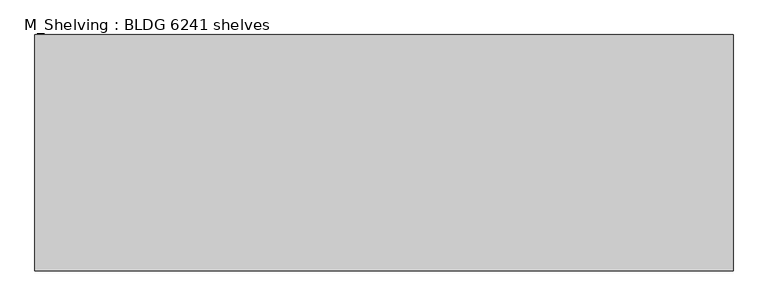
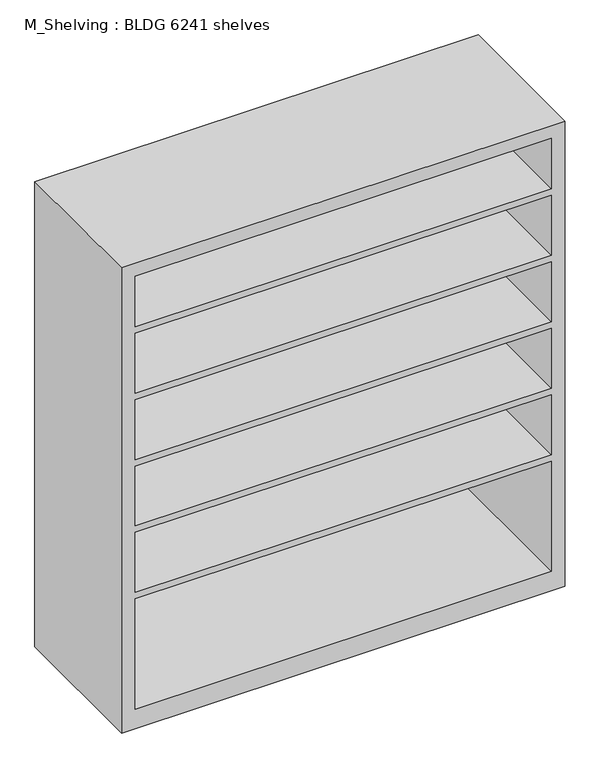
"""IFC4 building model written with IfcOpenShell, lengths in millimetres: furniture geometry, M_Shelving : BLDG 6241 shelves."""

from ifc_helpers import new_model, si_unit, frame, origin, place, context, project, spatial, polyline, outline, extrude, source, transform, mapped, element, save


def m_shelving_bldg_6241_shelves_72ad7da8(model_context):
    return source(origin(), model_context, "Body", "SweptSolid", [
        extrude(outline(polyline([(0.0, 825.5), (1830.0, 825.5), (1830.0, -825.5), (0.0, -825.5), (0.0, 825.5)]), holes=[polyline([(1779.2, 774.7), (1581.2714286, 774.7), (1581.2714286, -774.7), (1779.2, -774.7), (1779.2, 774.7)]), polyline([(76.2, 774.7), (76.2, -774.7), (510.1571429, -774.7), (510.1571429, 774.7), (76.2, 774.7)]), polyline([(1058.4142857, -774.7), (1294.4428571, -774.7), (1294.4428571, 774.7), (1058.4142857, 774.7), (1058.4142857, -774.7)]), polyline([(1555.8714286, 774.7), (1319.8428571, 774.7), (1319.8428571, -774.7), (1555.8714286, -774.7), (1555.8714286, 774.7)]), polyline([(1033.0142857, 774.7), (796.9857143, 774.7), (796.9857143, -774.7), (1033.0142857, -774.7), (1033.0142857, 774.7)]), polyline([(771.5857143, 774.7), (535.5571429, 774.7), (535.5571429, -774.7), (771.5857143, -774.7), (771.5857143, 774.7)])]), frame((0.0, -584.2, 0.0), z_axis=(0.0, 1.0, 0.0), x_axis=(0.0, 0.0, 1.0)), (0.0, 0.0, 1.0), 558.8),
    ])


if __name__ == "__main__":
    model = new_model("IFC4")
    model_context = context("Model", 3, world=origin())
    ifc_project = project(units=[si_unit("LENGTHUNIT", "METRE", prefix="MILLI")], contexts=[model_context])
    site = spatial("IfcSite", under=ifc_project)
    building = spatial("IfcBuilding", under=site)
    placement = place(None, origin())
    m_shelving_bldg_6241_shelves_shape = m_shelving_bldg_6241_shelves_72ad7da8(model_context)
    element("IfcFurniture", 1, ObjectType="M_Shelving : BLDG 6241 shelves", at=placement, inside=building, context=model_context, shape_type="MappedRepresentation", body=[
        mapped(m_shelving_bldg_6241_shelves_shape, transform((0.0, 0.0, 0.0), x_axis=(1.0, 0.0, 0.0), y_axis=(0.0, 1.0, 0.0), z_axis=(0.0, 0.0, 1.0))),
    ])
    save(model, "model.ifc")

# Revit data of these elements
# Type "M_Shelving : BLDG 6241 shelves"
#   Depth = 1' - 10"
#   Height = 6' - 0.04724"
#   Width = 5' - 5"
#   Material = Birch
#   Default Elevation = 0
# Element 1 (IfcFurniture, "M_Shelving : BLDG 6241 shelves")
#   Materials on its faces: "Birch"
# Materials
#   "Birch": class "Wood", colour RGB 224 178 126, transparency 0, Description = "Betula Alleghaniensis", Cost = 0
